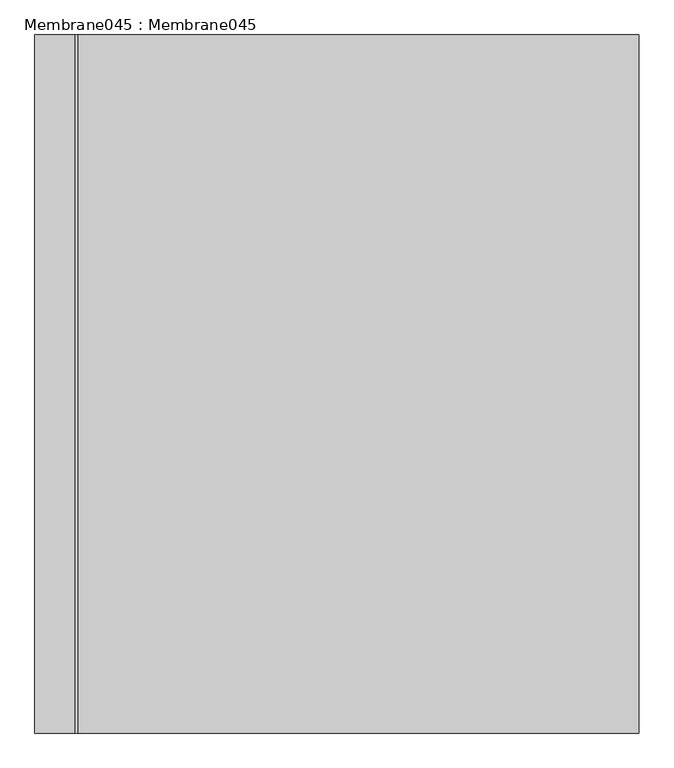
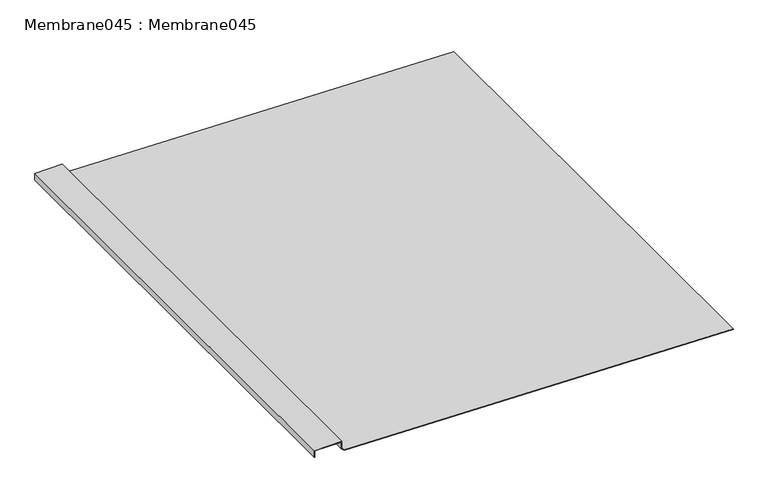
"""IFC4 building model written with IfcOpenShell, lengths in millimetres: proxy geometry, Membrane045 : Membrane045."""

from ifc_helpers import new_model, si_unit, frame, origin, place, context, project, spatial, polyline, outline, extrude, source, transform, mapped, element, save


def membrane045_membrane045_d5267264(model_context):
    return source(origin(), model_context, "Body", "SweptSolid", [
        extrude(outline(polyline([(40091.7340878, -5498.6781385), (40125.3341265, -7106.245476), (40135.5689314, -7116.3154297), (40165.4960083, -7116.3154297), (40165.4960083, -7230.3012695), (40136.1757812, -7230.3012695), (40136.1757812, -7228.3012695), (40163.4960083, -7228.3012695), (40163.4960083, -7118.3154297), (40134.75, -7118.3154297), (40123.3515625, -7107.1005859), (40089.7345245, -5498.7199317), (40091.7340878, -5498.6781385)])), frame((0.0, 7982.1531721, 0.0), z_axis=(0.0, 1.0, 0.0), x_axis=(0.0, 0.0, 1.0)), (0.0, 0.0, 1.0), 2000.0),
    ])


if __name__ == "__main__":
    model = new_model("IFC4")
    model_context = context("Model", 3, world=origin())
    ifc_project = project(units=[si_unit("LENGTHUNIT", "METRE", prefix="MILLI")], contexts=[model_context])
    site = spatial("IfcSite", under=ifc_project)
    building = spatial("IfcBuilding", under=site)
    placement = place(None, origin())
    membrane045_membrane045_shape = membrane045_membrane045_d5267264(model_context)
    element("IfcBuildingElementProxy", 1, Name="Membrane045 : Membrane045", ObjectType="Membrane045 : Membrane045", at=placement, inside=building, context=model_context, shape_type="MappedRepresentation", body=[
        mapped(membrane045_membrane045_shape, transform((0.0, 0.0, 0.0), x_axis=(1.0, 0.0, 0.0), y_axis=(0.0, 1.0, 0.0), z_axis=(0.0, 0.0, 1.0))),
    ])
    save(model, "model.ifc")

# Revit data of these elements
# Type "Membrane045 : Membrane045"
#   NameOverride = "Membrane045"
# Element 1 (IfcBuildingElementProxy, "Membrane045 : Membrane045")
#   Materials on its faces: "WESTCOAT ALX UNDER TILE WATERPROOFING SYSTEM (FOLLOW MANUFACTURER'S INSTALLATION REQUIREMENTS)"
# Materials
#   "WESTCOAT ALX UNDER TILE WATERPROOFING SYSTEM (FOLLOW MANUFACTURER'S INSTALLATION REQUIREMENTS)": class "Unassigned", colour RGB 27 232 0, transparency 0
